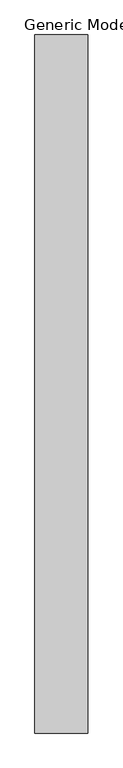
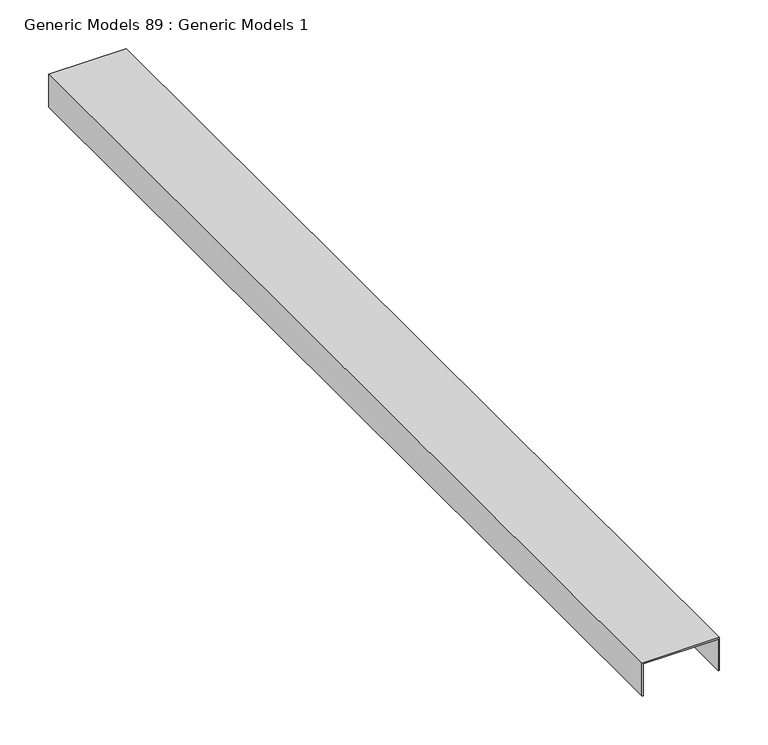
"""IFC4 building model written with IfcOpenShell, lengths in millimetres: proxy geometry, Generic Models 89 : Generic Models 1."""

import ifcopenshell
import ifcopenshell.guid

model = None  # the IFC model being written
_history = None  # IfcOwnerHistory: only IFC2X3 demands one
_inside = {}  # id of a spatial element -> (the spatial element, [elements in it])
_under = {}  # id of a project, library or spatial element -> (it, [spatial elements below it])
_declared = {}  # id of a project -> (the project, [libraries it declares])
_typed = {}  # id of a type object -> (the type object, [elements of that type])
_made_of = {}  # id of a material, layer set ... -> (it, [elements and type objects made of it])


def new_model(schema):
    """Start an empty IFC model of exactly this schema.

    Asked for "IFC4X3", IfcOpenShell would pick the latest addendum, in which some entities
    have other attributes; the version numbers below select the first issue.
    IFC2X3 requires an IfcOwnerHistory on every rooted entity: one is made here for all.
    """
    global model, _history
    if schema == "IFC4X3":
        model = ifcopenshell.file(schema_version=(4, 3, 0, 0))
    else:
        model = ifcopenshell.file(schema=schema)
    _inside.clear()
    _under.clear()
    _declared.clear()
    _typed.clear()
    _made_of.clear()
    _history = None
    if model.schema == "IFC2X3":
        org = make("IfcOrganization", Name="unknown")
        user = make(
            "IfcPersonAndOrganization",
            ThePerson=make("IfcPerson", FamilyName="unknown"),
            TheOrganization=org,
        )
        app = make(
            "IfcApplication",
            ApplicationDeveloper=org,
            Version="unknown",
            ApplicationFullName="unknown",
            ApplicationIdentifier="unknown",
        )
        _history = make(
            "IfcOwnerHistory",
            OwningUser=user,
            OwningApplication=app,
            ChangeAction="ADDED",
            CreationDate=0,
        )
    return model


def make(cls, **values):
    """One entity of the class cls with the attributes given. An attribute that is None is left unset."""
    return model.create_entity(
        cls, **{name: value for name, value in values.items() if value is not None}
    )


def rooted(cls, **values):
    """An entity with a GlobalId (a new one), such as an element, a storey or a relation."""
    return make(cls, GlobalId=ifcopenshell.guid.new(), OwnerHistory=_history, **values)


def si_unit(unit_type, name, prefix=None):
    """IfcSIUnit, for example si_unit("LENGTHUNIT", "METRE", prefix="MILLI")."""
    return make("IfcSIUnit", UnitType=unit_type, Prefix=prefix, Name=name)


def assignment(units):
    """IfcUnitAssignment: the units of a project."""
    return None if units is None else make("IfcUnitAssignment", Units=units)


def point(xyz):
    """IfcCartesianPoint."""
    return None if xyz is None else make("IfcCartesianPoint", Coordinates=xyz)


def direction(xyz):
    """IfcDirection."""
    return None if xyz is None else make("IfcDirection", DirectionRatios=xyz)


def frame(location, z_axis=None, x_axis=None):
    """IfcAxis2Placement3D, a coordinate frame: its origin and axes. An axis left out is left unset."""
    return make(
        "IfcAxis2Placement3D",
        Location=point(location),
        Axis=direction(z_axis),
        RefDirection=direction(x_axis),
    )


def origin():
    """The frame at (0, 0, 0) with its axes left unset."""
    return frame((0.0, 0.0, 0.0))


def place(relative_to, where):
    """IfcLocalPlacement: puts the frame where relative to a parent placement (None: the world)."""
    return make(
        "IfcLocalPlacement", PlacementRelTo=relative_to, RelativePlacement=where
    )


def context(
    kind, dimensions, precision=None, world=None, true_north=None, identifier=None
):
    """IfcGeometricRepresentationContext, for example the 3D "Model" context."""
    return make(
        "IfcGeometricRepresentationContext",
        ContextIdentifier=identifier,
        ContextType=kind,
        CoordinateSpaceDimension=dimensions,
        Precision=precision,
        WorldCoordinateSystem=world,
        TrueNorth=true_north,
    )


def project(units=None, contexts=None):
    """IfcProject with its units and contexts."""
    return rooted(
        "IfcProject",
        Name="project",
        RepresentationContexts=contexts,
        UnitsInContext=assignment(units),
    )


def spatial(cls, under=None, at=None, **own):
    """A site, building, storey or space (cls), placed at a placement, below another one or the project."""
    s = rooted(cls, ObjectPlacement=at, **own)
    if under is not None:
        _under.setdefault(under.id(), (under, []))[1].append(s)
    return s


def polyline(points):
    """IfcPolyline through the points."""
    return make("IfcPolyline", Points=[point(p) for p in points])


def outline(outer, holes=None, kind="AREA"):
    """IfcArbitraryClosedProfileDef: a profile drawn as a closed curve; with holes, ...WithVoids."""
    if holes is None:
        return make("IfcArbitraryClosedProfileDef", ProfileType=kind, OuterCurve=outer)
    return make(
        "IfcArbitraryProfileDefWithVoids",
        ProfileType=kind,
        OuterCurve=outer,
        InnerCurves=holes,
    )


def extrude(swept, where, along, depth):
    """IfcExtrudedAreaSolid: the profile swept, set in the frame where, extruded along a direction by depth."""
    return make(
        "IfcExtrudedAreaSolid",
        SweptArea=swept,
        Position=where,
        ExtrudedDirection=direction(along),
        Depth=depth,
    )


def shape(context_of_items, identifier, shape_type, items):
    """IfcShapeRepresentation: the items that make up one representation, for example the "Body"."""
    return make(
        "IfcShapeRepresentation",
        ContextOfItems=context_of_items,
        RepresentationIdentifier=identifier,
        RepresentationType=shape_type,
        Items=items,
    )


def source(mapping_origin, context_of_items, identifier, shape_type, items):
    """IfcRepresentationMap: a shape defined once, which mapped items show again and again."""
    return make(
        "IfcRepresentationMap",
        MappingOrigin=mapping_origin,
        MappedRepresentation=shape(context_of_items, identifier, shape_type, items),
    )


def transform(
    local_origin,
    x_axis=None,
    y_axis=None,
    z_axis=None,
    scale=None,
    scale2=None,
    scale3=None,
    uniform=True,
):
    """IfcCartesianTransformationOperator3D, or its non-uniform kind. x_axis, y_axis, z_axis: its Axis1, 2, 3."""
    if uniform:
        return make(
            "IfcCartesianTransformationOperator3D",
            Axis1=direction(x_axis),
            Axis2=direction(y_axis),
            LocalOrigin=point(local_origin),
            Scale=scale,
            Axis3=direction(z_axis),
        )
    return make(
        "IfcCartesianTransformationOperator3DnonUniform",
        Axis1=direction(x_axis),
        Axis2=direction(y_axis),
        LocalOrigin=point(local_origin),
        Scale=scale,
        Axis3=direction(z_axis),
        Scale2=scale2,
        Scale3=scale3,
    )


def mapped(mapping_source, mapping_target):
    """IfcMappedItem: shows the shape of a source again, moved by a transform."""
    return make(
        "IfcMappedItem", MappingSource=mapping_source, MappingTarget=mapping_target
    )


def made_of(thing, what):
    """Note that an element or type object is made of a material, layer set ...; save() writes the relation."""
    if what is not None:
        _made_of.setdefault(what.id(), (what, []))[1].append(thing)
    return thing


def element(
    cls,
    number,
    at=None,
    inside=None,
    cuts=None,
    type_object=None,
    material=None,
    context=None,
    identifier="Body",
    shape_type=None,
    held_by="IfcProductDefinitionShape",
    body=None,
    shapes=None,
    **own,
):
    """One element of the class cls, such as IfcWall. Its Tag is "e" and its number.

    at: its placement. inside: the storey or other place that contains it. cuts: it is an
    opening in that element (IfcRelVoidsElement). A single representation is given by context,
    identifier, shape_type and body (its items); several are given by shapes. held_by: the class
    of the entity that holds the representations. save() writes the other relations.
    """
    e = rooted(cls, Tag="e%d" % number, ObjectPlacement=at, **own)
    if body is not None:
        shapes = [shape(context, identifier, shape_type, body)]
    if shapes is not None:
        e.Representation = make(held_by, Representations=shapes)
    if inside is not None:
        _inside.setdefault(inside.id(), (inside, []))[1].append(e)
    if cuts is not None:
        rooted(
            "IfcRelVoidsElement", RelatingBuildingElement=cuts, RelatedOpeningElement=e
        )
    if type_object is not None:
        _typed.setdefault(type_object.id(), (type_object, []))[1].append(e)
    return made_of(e, material)


def aggregate(whole, parts):
    """IfcRelAggregates: a whole, such as a stair, and the parts it consists of."""
    return rooted("IfcRelAggregates", RelatingObject=whole, RelatedObjects=parts)


def save(model, path):
    """Write the relations noted so far, then the file.

    IfcRelAggregates (storeys below a building ...), IfcRelContainedInSpatialStructure (elements
    in a storey), IfcRelDefinesByType, IfcRelAssociatesMaterial and IfcRelDeclares: one each for
    every whole, place, type object, material and project.
    """
    for whole, parts in _under.values():
        aggregate(whole, parts)
    for where, things in _inside.values():
        rooted(
            "IfcRelContainedInSpatialStructure",
            RelatedElements=things,
            RelatingStructure=where,
        )
    for kind, things in _typed.values():
        rooted("IfcRelDefinesByType", RelatedObjects=things, RelatingType=kind)
    for what, things in _made_of.values():
        rooted("IfcRelAssociatesMaterial", RelatedObjects=things, RelatingMaterial=what)
    for by, libraries in _declared.values():
        rooted("IfcRelDeclares", RelatingContext=by, RelatedDefinitions=libraries)
    model.write(path)


def generic_models_89_generic_models_1_86fe7b68(model_context):
    return source(origin(), model_context, "Body", "SweptSolid", [
        extrude(outline(polyline([(2218.773933, 45716.6735531), (2218.773933, 45624.5985531), (2177.498933, 45624.5985531), (2177.498933, 45626.1860531), (2217.186433, 45626.1860531), (2217.186433, 45715.0860531), (2177.498933, 45715.0860531), (2177.498933, 45716.6735531), (2218.773933, 45716.6735531)])), frame((0.0, 0.0, 0.0), z_axis=(0.0, 1.0, 0.0), x_axis=(0.0, 0.0, 1.0)), (0.0, 0.0, 1.0), 1219.2),
    ])


if __name__ == "__main__":
    model = new_model("IFC4")
    model_context = context("Model", 3, world=origin())
    ifc_project = project(units=[si_unit("LENGTHUNIT", "METRE", prefix="MILLI")], contexts=[model_context])
    site = spatial("IfcSite", under=ifc_project)
    building = spatial("IfcBuilding", under=site)
    placement = place(None, origin())
    generic_models_89_generic_models_1_shape = generic_models_89_generic_models_1_86fe7b68(model_context)
    element("IfcBuildingElementProxy", 1, Name="Generic Models 89 : Generic Models 1", ObjectType="Generic Models 89 : Generic Models 1", at=placement, inside=building, context=model_context, shape_type="MappedRepresentation", body=[
        mapped(generic_models_89_generic_models_1_shape, transform((0.0, 0.0, 0.0), x_axis=(1.0, 0.0, 0.0), y_axis=(0.0, 1.0, 0.0), z_axis=(0.0, 0.0, 1.0))),
    ])
    save(model, "model.ifc")

# Revit data of these elements
# Element 1 (IfcBuildingElementProxy, "Generic Models 89 : Generic Models 1")
#   Materials on its faces: "METAL RUNNER CHANNEL TO RUN CONTINOUS FROM WALL TO WALL (ANCHOR AT BOTH ENDS)"
# Materials
#   "METAL RUNNER CHANNEL TO RUN CONTINOUS FROM WALL TO WALL (ANCHOR AT BOTH ENDS)": class "Unassigned", colour RGB 210 209 208, transparency 0, Keynote = "M05121300.02", Cost = 0
